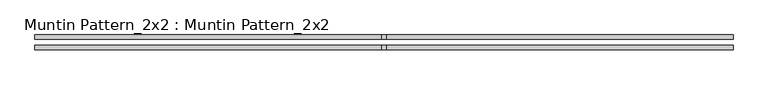
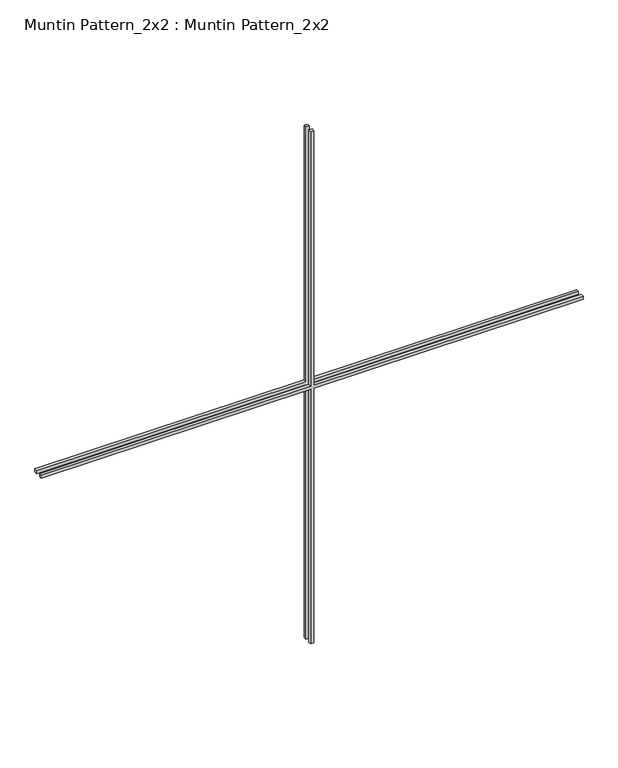
"""IFC4 building model written with IfcOpenShell, lengths in millimetres: proxy geometry, Muntin Pattern_2x2 : Muntin Pattern_2x2."""

from ifc_helpers import new_model, si_unit, frame, origin, place, context, project, spatial, polyline, outline, extrude, source, transform, mapped, element, save


def muntin_pattern_2x2_muntin_pattern_2x2_b1a79f21(model_context):
    return source(origin(), model_context, "Body", "SweptSolid", [
        extrude(outline(polyline([(1068.25, -6.35), (1068.25, -1061.9), (1055.55, -1061.9), (1055.55, -6.35), (0.0, -6.35), (0.0, 6.35), (1055.55, 6.35), (1055.55, 1061.9), (1068.25, 1061.9), (1068.25, 6.35), (2123.8, 6.35), (2123.8, -6.35), (1068.25, -6.35)])), frame((0.0, -22.225, 0.0), z_axis=(0.0, 1.0, 0.0), x_axis=(0.0, 0.0, 1.0)), (0.0, 0.0, 1.0), 12.7),
        extrude(outline(polyline([(1068.25, -6.35), (1068.25, -1061.9), (1055.55, -1061.9), (1055.55, -6.35), (0.0, -6.35), (0.0, 6.35), (1055.55, 6.35), (1055.55, 1061.9), (1068.25, 1061.9), (1068.25, 6.35), (2123.8, 6.35), (2123.8, -6.35), (1068.25, -6.35)])), frame((0.0, 9.525, 0.0), z_axis=(0.0, 1.0, 0.0), x_axis=(0.0, 0.0, 1.0)), (0.0, 0.0, 1.0), 12.7),
    ])


if __name__ == "__main__":
    model = new_model("IFC4")
    model_context = context("Model", 3, world=origin())
    ifc_project = project(units=[si_unit("LENGTHUNIT", "METRE", prefix="MILLI")], contexts=[model_context])
    site = spatial("IfcSite", under=ifc_project)
    building = spatial("IfcBuilding", under=site)
    placement = place(None, origin())
    muntin_pattern_2x2_muntin_pattern_2x2_shape = muntin_pattern_2x2_muntin_pattern_2x2_b1a79f21(model_context)
    element("IfcBuildingElementProxy", 1, Name="Muntin Pattern_2x2 : Muntin Pattern_2x2", ObjectType="Muntin Pattern_2x2 : Muntin Pattern_2x2", at=placement, inside=building, context=model_context, shape_type="MappedRepresentation", body=[
        mapped(muntin_pattern_2x2_muntin_pattern_2x2_shape, transform((0.0, 0.0, 0.0), x_axis=(1.0, 0.0, 0.0), y_axis=(0.0, 1.0, 0.0), z_axis=(0.0, 0.0, 1.0))),
    ])
    save(model, "model.ifc")

# Revit data of these elements
# Type "Muntin Pattern_2x2 : Muntin Pattern_2x2"
#   Width [instance default] = 1.2192 m
#   Thickness = 0.0127 m
#   Height [instance default] = 1.2192 m
#   Distance = 0.01905 m
#   Interior Material [instance default] = none
#   Exterior Material [instance default] = none
#   Default Elevation = 0
# Element 1 (IfcBuildingElementProxy, "Muntin Pattern_2x2 : Muntin Pattern_2x2")
#   Width = 2.1238 m
#   Height = 2.1238 m
#   Interior Material = Wood - Stained
#   Exterior Material = Clad - White
#   Materials on its faces: "Clad - White", "Wood - Stained"
# Materials
#   "Clad - White": class "Wood", colour RGB 242 242 238, transparency 0, Cost = 0
#   "Wood - Stained": class "Wood", colour RGB 227 170 128, transparency 0, Cost = 0
